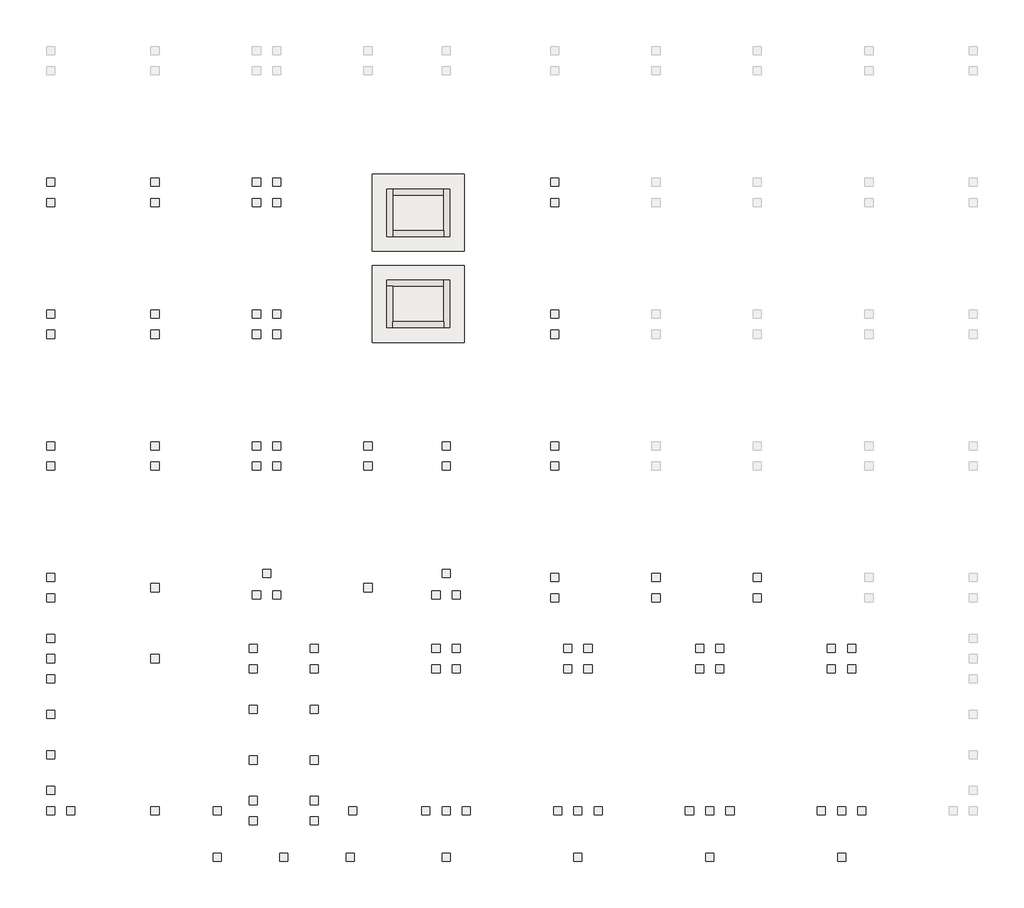
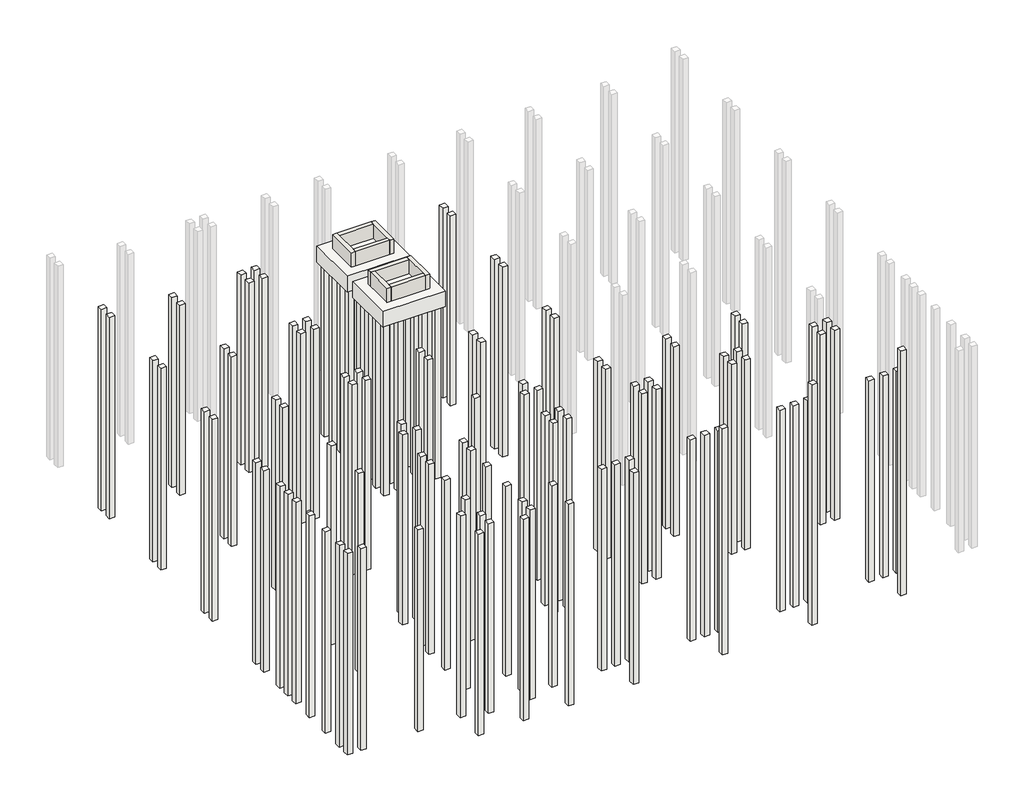
# Not in any storey, part 1 of 2: 143 footings, 8 walls.
# Revit data of these elements (continued)
# Type "NLRS_17_SFO_TLB_funderingspaal geheid beton prefab-AV-MMBPC_gen_rsf : heipaal beton prefab_gen__bxh 400x400"
#   IfcExportAs = "IfcPile"
#   Type Comments = "prefab heipaal 400x400"
#   Model = " "
#   Manufacturer = " "
#   Description = "prefab heipaal 400x400"
#   Assembly Code = "17.21"
#   Width = 400 mm
#   Slanted Angle [instance default] = 0.00°
#   NLRS_S_draagvermogen_trek [instance default] = 0.00 kN
#   NLRS_S_draagvermogen_druk [instance default] = 0.00 kN
#   NLRS_C_lengte [instance default] = 1660 mm
#   NLRS_C_hoogte = 400 mm
#   NLRS_C_breedte = 400 mm
#   Height [instance default] = 1660 mm
#   Length [instance default] = 1660 mm
#   Angle [instance default] = 0.00°
#   Slanted [instance default] = 0
#   Structural Material = NLRS_f2_beton prefab_gen_rsf
#   Keynote = ""
# Type "NLRS_16_WA_beton ihw 300_gen_rsf"
#   Keynote = ""
#   Type IfcGUID = "3S1HfGygHC08_ZXeiJ7DHR"
#   Description = "buitenwand beton ihw, generiek"
#   Assembly Code = "16.23"
#   IfcExportAs = "IfcWall"
#   Layers, outside or top first: 300 mm "NLRS_f2_beton ihwg_gen_rsf" (function 1)
# Element 1 (IfcFooting, "NLRS_16_SFO_LB_funderingspoer meerpaals beton ihwg-MMBC-SH_gen_rsf : funderingspoer beton ihwg_gen__lift bxlxh 3800x4550x1200")
#   IfcGUID = "22y6L5gAz9AR8RjJaZzOwK"
#   Height = 1200 mm
#   Depth = 0 mm
#   IsExternal = yes
#   LoadBearing = yes
#   Phase Created = NLRS_nieuw
#   Materials on its faces: "NLRS_f2_beton ihwg_gen_rsf"
# Element 2 (IfcFooting, "NLRS_16_SFO_LB_funderingspoer meerpaals beton ihwg-MMBC-SH_gen_rsf : funderingspoer beton ihwg_gen__lift bxlxh 3800x4550x1200")
#   IfcGUID = "22y6L5gAz9AR8RjJaZzOui"
#   Height = 1200 mm
#   Depth = 0 mm
#   IsExternal = yes
#   LoadBearing = yes
#   Phase Created = NLRS_nieuw
#   Materials on its faces: "NLRS_f2_beton ihwg_gen_rsf"
# Element 3 (IfcFooting, "NLRS_17_SFO_TLB_funderingspaal geheid beton prefab-AV-MMBPC_gen_rsf : heipaal beton prefab_gen__bxh 400x400")
#   IfcGUID = "10$Kfo5uPCAOPJEOo5LEvz"
#   Slanted Angle = 0.00°
#   NLRS_S_draagvermogen_trek = 0.00 kN
#   NLRS_S_draagvermogen_druk = 0.00 kN
#   Angle = 0.00°
#   IsExternal = yes
#   LoadBearing = yes
#   Slanted = 0
#   Phase Created = NLRS_nieuw
#   Materials on its faces: "NLRS_f2_beton prefab_gen_rsf"
# Element 4 (IfcFooting, "NLRS_17_SFO_TLB_funderingspaal geheid beton prefab-AV-MMBPC_gen_rsf : heipaal beton prefab_gen__bxh 400x400")
#   IfcGUID = "10$Kfo5uPCAOPJEOo5LEuK"
#   Slanted Angle = 0.00°
#   NLRS_S_draagvermogen_trek = 0.00 kN
#   NLRS_S_draagvermogen_druk = 0.00 kN
#   Angle = 0.00°
#   IsExternal = yes
#   LoadBearing = yes
#   Slanted = 0
#   Phase Created = NLRS_nieuw
#   Materials on its faces: "NLRS_f2_beton prefab_gen_rsf"
# Element 5 (IfcFooting, "NLRS_17_SFO_TLB_funderingspaal geheid beton prefab-AV-MMBPC_gen_rsf : heipaal beton prefab_gen__bxh 400x400")
#   IfcGUID = "10$Kfo5uPCAOPJEOo5LEuY"
#   Slanted Angle = 0.00°
#   NLRS_S_draagvermogen_trek = 0.00 kN
#   NLRS_S_draagvermogen_druk = 0.00 kN
#   Angle = 0.00°
#   IsExternal = yes
#   LoadBearing = yes
#   Slanted = 0
#   Phase Created = NLRS_nieuw
#   Materials on its faces: "NLRS_f2_beton prefab_gen_rsf"
# Element 6 (IfcFooting, "NLRS_17_SFO_TLB_funderingspaal geheid beton prefab-AV-MMBPC_gen_rsf : heipaal beton prefab_gen__bxh 400x400")
#   IfcGUID = "10$Kfo5uPCAOPJEOo5LEu$"
#   Slanted Angle = 0.00°
#   NLRS_S_draagvermogen_trek = 0.00 kN
#   NLRS_S_draagvermogen_druk = 0.00 kN
#   Angle = 0.00°
#   IsExternal = yes
#   LoadBearing = yes
#   Slanted = 0
#   Phase Created = NLRS_nieuw
#   Materials on its faces: "NLRS_f2_beton prefab_gen_rsf"
# Element 7 (IfcFooting, "NLRS_17_SFO_TLB_funderingspaal geheid beton prefab-AV-MMBPC_gen_rsf : heipaal beton prefab_gen__bxh 400x400")
#   IfcGUID = "10$Kfo5uPCAOPJEOo5LEun"
#   Slanted Angle = 0.00°
#   NLRS_S_draagvermogen_trek = 0.00 kN
#   NLRS_S_draagvermogen_druk = 0.00 kN
#   Angle = 0.00°
#   IsExternal = yes
#   LoadBearing = yes
#   Slanted = 0
#   Phase Created = NLRS_nieuw
#   Materials on its faces: "NLRS_f2_beton prefab_gen_rsf"
# Element 8 (IfcFooting, "NLRS_17_SFO_TLB_funderingspaal geheid beton prefab-AV-MMBPC_gen_rsf : heipaal beton prefab_gen__bxh 400x400")
#   IfcGUID = "10$Kfo5uPCAOPJEOo5LEtC"
#   Slanted Angle = 0.00°
#   NLRS_S_draagvermogen_trek = 0.00 kN
#   NLRS_S_draagvermogen_druk = 0.00 kN
#   Angle = 0.00°
#   IsExternal = yes
#   LoadBearing = yes
#   Slanted = 0
#   Phase Created = NLRS_nieuw
#   Materials on its faces: "NLRS_f2_beton prefab_gen_rsf"
# Element 9 (IfcFooting, "NLRS_17_SFO_TLB_funderingspaal geheid beton prefab-AV-MMBPC_gen_rsf : heipaal beton prefab_gen__bxh 400x400")
#   IfcGUID = "10$Kfo5uPCAOPJEOo5LEtE"
#   Slanted Angle = 0.00°
#   NLRS_S_draagvermogen_trek = 0.00 kN
#   NLRS_S_draagvermogen_druk = 0.00 kN
#   Angle = 0.00°
#   IsExternal = yes
#   LoadBearing = yes
#   Slanted = 0
#   Phase Created = NLRS_nieuw
#   Materials on its faces: "NLRS_f2_beton prefab_gen_rsf"
# Element 10 (IfcFooting, "NLRS_17_SFO_TLB_funderingspaal geheid beton prefab-AV-MMBPC_gen_rsf : heipaal beton prefab_gen__bxh 400x400")
#   IfcGUID = "10$Kfo5uPCAOPJEOo5LEtR"
#   Slanted Angle = 0.00°
#   NLRS_S_draagvermogen_trek = 0.00 kN
#   NLRS_S_draagvermogen_druk = 0.00 kN
#   Angle = 0.00°
#   IsExternal = yes
#   LoadBearing = yes
#   Slanted = 0
#   Phase Created = NLRS_nieuw
#   Materials on its faces: "NLRS_f2_beton prefab_gen_rsf"
# Element 11 (IfcFooting, "NLRS_17_SFO_TLB_funderingspaal geheid beton prefab-AV-MMBPC_gen_rsf : heipaal beton prefab_gen__bxh 400x400")
#   IfcGUID = "10$Kfo5uPCAOPJEOo5LEtT"
#   Slanted Angle = 0.00°
#   NLRS_S_draagvermogen_trek = 0.00 kN
#   NLRS_S_draagvermogen_druk = 0.00 kN
#   Angle = 0.00°
#   IsExternal = yes
#   LoadBearing = yes
#   Slanted = 0
#   Phase Created = NLRS_nieuw
#   Materials on its faces: "NLRS_f2_beton prefab_gen_rsf"
# Element 12 (IfcFooting, "NLRS_17_SFO_TLB_funderingspaal geheid beton prefab-AV-MMBPC_gen_rsf : heipaal beton prefab_gen__bxh 400x400")
#   IfcGUID = "10$Kfo5uPCAOPJEOo5LEte"
#   Slanted Angle = 0.00°
#   NLRS_S_draagvermogen_trek = 0.00 kN
#   NLRS_S_draagvermogen_druk = 0.00 kN
#   Angle = 0.00°
#   IsExternal = yes
#   LoadBearing = yes
#   Slanted = 0
#   Phase Created = NLRS_nieuw
#   Materials on its faces: "NLRS_f2_beton prefab_gen_rsf"
# Element 13 (IfcFooting, "NLRS_17_SFO_TLB_funderingspaal geheid beton prefab-AV-MMBPC_gen_rsf : heipaal beton prefab_gen__bxh 400x400")
#   IfcGUID = "10$Kfo5uPCAOPJEOo5LEtg"
#   Slanted Angle = 0.00°
#   NLRS_S_draagvermogen_trek = 0.00 kN
#   NLRS_S_draagvermogen_druk = 0.00 kN
#   Angle = 0.00°
#   IsExternal = yes
#   LoadBearing = yes
#   Slanted = 0
#   Phase Created = NLRS_nieuw
#   Materials on its faces: "NLRS_f2_beton prefab_gen_rsf"
# Element 14 (IfcFooting, "NLRS_17_SFO_TLB_funderingspaal geheid beton prefab-AV-MMBPC_gen_rsf : heipaal beton prefab_gen__bxh 400x400")
#   IfcGUID = "10$Kfo5uPCAOPJEOo5LEtb"
#   Slanted Angle = 0.00°
#   NLRS_S_draagvermogen_trek = 0.00 kN
#   NLRS_S_draagvermogen_druk = 0.00 kN
#   Angle = 0.00°
#   IsExternal = yes
#   LoadBearing = yes
#   Slanted = 0
#   Phase Created = NLRS_nieuw
#   Materials on its faces: "NLRS_f2_beton prefab_gen_rsf"
# Element 15 (IfcFooting, "NLRS_17_SFO_TLB_funderingspaal geheid beton prefab-AV-MMBPC_gen_rsf : heipaal beton prefab_gen__bxh 400x400")
#   IfcGUID = "10$Kfo5uPCAOPJEOo5LEtd"
#   Slanted Angle = 0.00°
#   NLRS_S_draagvermogen_trek = 0.00 kN
#   NLRS_S_draagvermogen_druk = 0.00 kN
#   Angle = 0.00°
#   IsExternal = yes
#   LoadBearing = yes
#   Slanted = 0
#   Phase Created = NLRS_nieuw
#   Materials on its faces: "NLRS_f2_beton prefab_gen_rsf"
# Element 16 (IfcFooting, "NLRS_17_SFO_TLB_funderingspaal geheid beton prefab-AV-MMBPC_gen_rsf : heipaal beton prefab_gen__bxh 400x400")
#   IfcGUID = "10$Kfo5uPCAOPJEOo5LEsp"
#   Slanted Angle = 0.00°
#   NLRS_S_draagvermogen_trek = 0.00 kN
#   NLRS_S_draagvermogen_druk = 0.00 kN
#   Angle = 0.00°
#   IsExternal = yes
#   LoadBearing = yes
#   Slanted = 0
#   Phase Created = NLRS_nieuw
#   Materials on its faces: "NLRS_f2_beton prefab_gen_rsf"
# Element 17 (IfcFooting, "NLRS_17_SFO_TLB_funderingspaal geheid beton prefab-AV-MMBPC_gen_rsf : heipaal beton prefab_gen__bxh 400x400")
#   IfcGUID = "10$Kfo5uPCAOPJEOo5LEsr"
#   Slanted Angle = 0.00°
#   NLRS_S_draagvermogen_trek = 0.00 kN
#   NLRS_S_draagvermogen_druk = 0.00 kN
#   Angle = 0.00°
#   IsExternal = yes
#   LoadBearing = yes
#   Slanted = 0
#   Phase Created = NLRS_nieuw
#   Materials on its faces: "NLRS_f2_beton prefab_gen_rsf"
# Element 18 (IfcFooting, "NLRS_17_SFO_TLB_funderingspaal geheid beton prefab-AV-MMBPC_gen_rsf : heipaal beton prefab_gen__bxh 400x400")
#   IfcGUID = "10$Kfo5uPCAOPJEOo5LEr0"
#   Slanted Angle = 0.00°
#   NLRS_S_draagvermogen_trek = 0.00 kN
#   NLRS_S_draagvermogen_druk = 0.00 kN
#   Angle = 0.00°
#   IsExternal = yes
#   LoadBearing = yes
#   Slanted = 0
#   Phase Created = NLRS_nieuw
#   Materials on its faces: "NLRS_f2_beton prefab_gen_rsf"
# Element 19 (IfcFooting, "NLRS_17_SFO_TLB_funderingspaal geheid beton prefab-AV-MMBPC_gen_rsf : heipaal beton prefab_gen__bxh 400x400")
#   IfcGUID = "10$Kfo5uPCAOPJEOo5LEr2"
#   Slanted Angle = 0.00°
#   NLRS_S_draagvermogen_trek = 0.00 kN
#   NLRS_S_draagvermogen_druk = 0.00 kN
#   Angle = 0.00°
#   IsExternal = yes
#   LoadBearing = yes
#   Slanted = 0
#   Phase Created = NLRS_nieuw
#   Materials on its faces: "NLRS_f2_beton prefab_gen_rsf"
# Element 20 (IfcFooting, "NLRS_17_SFO_TLB_funderingspaal geheid beton prefab-AV-MMBPC_gen_rsf : heipaal beton prefab_gen__bxh 400x400")
#   IfcGUID = "10$Kfo5uPCAOPJEOo5LErR"
#   Slanted Angle = 0.00°
#   NLRS_S_draagvermogen_trek = 0.00 kN
#   NLRS_S_draagvermogen_druk = 0.00 kN
#   Angle = 0.00°
#   IsExternal = yes
#   LoadBearing = yes
#   Slanted = 0
#   Phase Created = NLRS_nieuw
#   Materials on its faces: "NLRS_f2_beton prefab_gen_rsf"
# Element 21 (IfcFooting, "NLRS_17_SFO_TLB_funderingspaal geheid beton prefab-AV-MMBPC_gen_rsf : heipaal beton prefab_gen__bxh 400x400")
#   IfcGUID = "10$Kfo5uPCAOPJEOo5LErT"
#   Slanted Angle = 0.00°
#   NLRS_S_draagvermogen_trek = 0.00 kN
#   NLRS_S_draagvermogen_druk = 0.00 kN
#   Angle = 0.00°
#   IsExternal = yes
#   LoadBearing = yes
#   Slanted = 0
#   Phase Created = NLRS_nieuw
#   Materials on its faces: "NLRS_f2_beton prefab_gen_rsf"
# Element 22 (IfcFooting, "NLRS_17_SFO_TLB_funderingspaal geheid beton prefab-AV-MMBPC_gen_rsf : heipaal beton prefab_gen__bxh 400x400")
#   IfcGUID = "10$Kfo5uPCAOPJEOo5LErd"
#   Slanted Angle = 0.00°
#   NLRS_S_draagvermogen_trek = 0.00 kN
#   NLRS_S_draagvermogen_druk = 0.00 kN
#   Angle = 0.00°
#   IsExternal = yes
#   LoadBearing = yes
#   Slanted = 0
#   Phase Created = NLRS_nieuw
#   Materials on its faces: "NLRS_f2_beton prefab_gen_rsf"
# Element 23 (IfcFooting, "NLRS_17_SFO_TLB_funderingspaal geheid beton prefab-AV-MMBPC_gen_rsf : heipaal beton prefab_gen__bxh 400x400")
#   IfcGUID = "10$Kfo5uPCAOPJEOo5LErv"
#   Slanted Angle = 0.00°
#   NLRS_S_draagvermogen_trek = 0.00 kN
#   NLRS_S_draagvermogen_druk = 0.00 kN
#   Angle = 0.00°
#   IsExternal = yes
#   LoadBearing = yes
#   Slanted = 0
#   Phase Created = NLRS_nieuw
#   Materials on its faces: "NLRS_f2_beton prefab_gen_rsf"
# Element 24 (IfcFooting, "NLRS_17_SFO_TLB_funderingspaal geheid beton prefab-AV-MMBPC_gen_rsf : heipaal beton prefab_gen__bxh 400x400")
#   IfcGUID = "10$Kfo5uPCAOPJEOo5LEq5"
#   Slanted Angle = 0.00°
#   NLRS_S_draagvermogen_trek = 0.00 kN
#   NLRS_S_draagvermogen_druk = 0.00 kN
#   Angle = 0.00°
#   IsExternal = yes
#   LoadBearing = yes
#   Slanted = 0
#   Phase Created = NLRS_nieuw
#   Materials on its faces: "NLRS_f2_beton prefab_gen_rsf"
# Element 25 (IfcFooting, "NLRS_17_SFO_TLB_funderingspaal geheid beton prefab-AV-MMBPC_gen_rsf : heipaal beton prefab_gen__bxh 400x400")
#   IfcGUID = "10$Kfo5uPCAOPJEOo5LEq7"
#   Slanted Angle = 0.00°
#   NLRS_S_draagvermogen_trek = 0.00 kN
#   NLRS_S_draagvermogen_druk = 0.00 kN
#   Angle = 0.00°
#   IsExternal = yes
#   LoadBearing = yes
#   Slanted = 0
#   Phase Created = NLRS_nieuw
#   Materials on its faces: "NLRS_f2_beton prefab_gen_rsf"
# Element 26 (IfcFooting, "NLRS_17_SFO_TLB_funderingspaal geheid beton prefab-AV-MMBPC_gen_rsf : heipaal beton prefab_gen__bxh 400x400")
#   IfcGUID = "10$Kfo5uPCAOPJEOo5LEqa"
#   Slanted Angle = 0.00°
#   NLRS_S_draagvermogen_trek = 0.00 kN
#   NLRS_S_draagvermogen_druk = 0.00 kN
#   Angle = 0.00°
#   IsExternal = yes
#   LoadBearing = yes
#   Slanted = 0
#   Phase Created = NLRS_nieuw
#   Materials on its faces: "NLRS_f2_beton prefab_gen_rsf"
# Element 27 (IfcFooting, "NLRS_17_SFO_TLB_funderingspaal geheid beton prefab-AV-MMBPC_gen_rsf : heipaal beton prefab_gen__bxh 400x400")
#   IfcGUID = "10$Kfo5uPCAOPJEOo5LEqc"
#   Slanted Angle = 0.00°
#   NLRS_S_draagvermogen_trek = 0.00 kN
#   NLRS_S_draagvermogen_druk = 0.00 kN
#   Angle = 0.00°
#   IsExternal = yes
#   LoadBearing = yes
#   Slanted = 0
#   Phase Created = NLRS_nieuw
#   Materials on its faces: "NLRS_f2_beton prefab_gen_rsf"
# Element 28 (IfcFooting, "NLRS_17_SFO_TLB_funderingspaal geheid beton prefab-AV-MMBPC_gen_rsf : heipaal beton prefab_gen__bxh 400x400")
#   IfcGUID = "10$Kfo5uPCAOPJEOo5LEqy"
#   Slanted Angle = 0.00°
#   NLRS_S_draagvermogen_trek = 0.00 kN
#   NLRS_S_draagvermogen_druk = 0.00 kN
#   Angle = 0.00°
#   IsExternal = yes
#   LoadBearing = yes
#   Slanted = 0
#   Phase Created = NLRS_nieuw
#   Materials on its faces: "NLRS_f2_beton prefab_gen_rsf"
# Element 29 (IfcFooting, "NLRS_17_SFO_TLB_funderingspaal geheid beton prefab-AV-MMBPC_gen_rsf : heipaal beton prefab_gen__bxh 400x400")
#   IfcGUID = "10$Kfo5uPCAOPJEOo5LEq_"
#   Slanted Angle = 0.00°
#   NLRS_S_draagvermogen_trek = 0.00 kN
#   NLRS_S_draagvermogen_druk = 0.00 kN
#   Angle = 0.00°
#   IsExternal = yes
#   LoadBearing = yes
#   Slanted = 0
#   Phase Created = NLRS_nieuw
#   Materials on its faces: "NLRS_f2_beton prefab_gen_rsf"
# Element 30 (IfcFooting, "NLRS_17_SFO_TLB_funderingspaal geheid beton prefab-AV-MMBPC_gen_rsf : heipaal beton prefab_gen__bxh 400x400")
#   IfcGUID = "10$Kfo5uPCAOPJEOo5LEpB"
#   Slanted Angle = 0.00°
#   NLRS_S_draagvermogen_trek = 0.00 kN
#   NLRS_S_draagvermogen_druk = 0.00 kN
#   Angle = 0.00°
#   IsExternal = yes
#   LoadBearing = yes
#   Slanted = 0
#   Phase Created = NLRS_nieuw
#   Materials on its faces: "NLRS_f2_beton prefab_gen_rsf"
# Element 31 (IfcFooting, "NLRS_17_SFO_TLB_funderingspaal geheid beton prefab-AV-MMBPC_gen_rsf : heipaal beton prefab_gen__bxh 400x400")
#   IfcGUID = "10$Kfo5uPCAOPJEOo5LEpD"
#   Slanted Angle = 0.00°
#   NLRS_S_draagvermogen_trek = 0.00 kN
#   NLRS_S_draagvermogen_druk = 0.00 kN
#   Angle = 0.00°
#   IsExternal = yes
#   LoadBearing = yes
#   Slanted = 0
#   Phase Created = NLRS_nieuw
#   Materials on its faces: "NLRS_f2_beton prefab_gen_rsf"
# Element 32 (IfcFooting, "NLRS_17_SFO_TLB_funderingspaal geheid beton prefab-AV-MMBPC_gen_rsf : heipaal beton prefab_gen__bxh 400x400")
#   IfcGUID = "10$Kfo5uPCAOPJEOo5LEp3"
#   Slanted Angle = 0.00°
#   NLRS_S_draagvermogen_trek = 0.00 kN
#   NLRS_S_draagvermogen_druk = 0.00 kN
#   Angle = 0.00°
#   IsExternal = yes
#   LoadBearing = yes
#   Slanted = 0
#   Phase Created = NLRS_nieuw
#   Materials on its faces: "NLRS_f2_beton prefab_gen_rsf"
# Element 33 (IfcFooting, "NLRS_17_SFO_TLB_funderingspaal geheid beton prefab-AV-MMBPC_gen_rsf : heipaal beton prefab_gen__bxh 400x400")
#   IfcGUID = "10$Kfo5uPCAOPJEOo5LEp5"
#   Slanted Angle = 0.00°
#   NLRS_S_draagvermogen_trek = 0.00 kN
#   NLRS_S_draagvermogen_druk = 0.00 kN
#   Angle = 0.00°
#   IsExternal = yes
#   LoadBearing = yes
#   Slanted = 0
#   Phase Created = NLRS_nieuw
#   Materials on its faces: "NLRS_f2_beton prefab_gen_rsf"
# Element 34 (IfcFooting, "NLRS_17_SFO_TLB_funderingspaal geheid beton prefab-AV-MMBPC_gen_rsf : heipaal beton prefab_gen__bxh 400x400")
#   IfcGUID = "10$Kfo5uPCAOPJEOo5LEpG"
#   Slanted Angle = 0.00°
#   NLRS_S_draagvermogen_trek = 0.00 kN
#   NLRS_S_draagvermogen_druk = 0.00 kN
#   Angle = 0.00°
#   IsExternal = yes
#   LoadBearing = yes
#   Slanted = 0
#   Phase Created = NLRS_nieuw
#   Materials on its faces: "NLRS_f2_beton prefab_gen_rsf"
# Element 35 (IfcFooting, "NLRS_17_SFO_TLB_funderingspaal geheid beton prefab-AV-MMBPC_gen_rsf : heipaal beton prefab_gen__bxh 400x400")
#   IfcGUID = "10$Kfo5uPCAOPJEOo5LEpI"
#   Slanted Angle = 0.00°
#   NLRS_S_draagvermogen_trek = 0.00 kN
#   NLRS_S_draagvermogen_druk = 0.00 kN
#   Angle = 0.00°
#   IsExternal = yes
#   LoadBearing = yes
#   Slanted = 0
#   Phase Created = NLRS_nieuw
#   Materials on its faces: "NLRS_f2_beton prefab_gen_rsf"
# Element 36 (IfcFooting, "NLRS_17_SFO_TLB_funderingspaal geheid beton prefab-AV-MMBPC_gen_rsf : heipaal beton prefab_gen__bxh 400x400")
#   IfcGUID = "10$Kfo5uPCAOPJEOo5LEpe"
#   Slanted Angle = 0.00°
#   NLRS_S_draagvermogen_trek = 0.00 kN
#   NLRS_S_draagvermogen_druk = 0.00 kN
#   Angle = 0.00°
#   IsExternal = yes
#   LoadBearing = yes
#   Slanted = 0
#   Phase Created = NLRS_nieuw
#   Materials on its faces: "NLRS_f2_beton prefab_gen_rsf"
# Element 37 (IfcFooting, "NLRS_17_SFO_TLB_funderingspaal geheid beton prefab-AV-MMBPC_gen_rsf : heipaal beton prefab_gen__bxh 400x400")
#   IfcGUID = "10$Kfo5uPCAOPJEOo5LEpg"
#   Slanted Angle = 0.00°
#   NLRS_S_draagvermogen_trek = 0.00 kN
#   NLRS_S_draagvermogen_druk = 0.00 kN
#   Angle = 0.00°
#   IsExternal = yes
#   LoadBearing = yes
#   Slanted = 0
#   Phase Created = NLRS_nieuw
#   Materials on its faces: "NLRS_f2_beton prefab_gen_rsf"
# Element 38 (IfcFooting, "NLRS_17_SFO_TLB_funderingspaal geheid beton prefab-AV-MMBPC_gen_rsf : heipaal beton prefab_gen__bxh 400x400")
#   IfcGUID = "10$Kfo5uPCAOPJEOo5LEoA"
#   Slanted Angle = 0.00°
#   NLRS_S_draagvermogen_trek = 0.00 kN
#   NLRS_S_draagvermogen_druk = 0.00 kN
#   Angle = 0.00°
#   IsExternal = yes
#   LoadBearing = yes
#   Slanted = 0
#   Phase Created = NLRS_nieuw
#   Materials on its faces: "NLRS_f2_beton prefab_gen_rsf"
# Element 39 (IfcFooting, "NLRS_17_SFO_TLB_funderingspaal geheid beton prefab-AV-MMBPC_gen_rsf : heipaal beton prefab_gen__bxh 400x400")
#   IfcGUID = "10$Kfo5uPCAOPJEOo5LEoC"
#   Slanted Angle = 0.00°
#   NLRS_S_draagvermogen_trek = 0.00 kN
#   NLRS_S_draagvermogen_druk = 0.00 kN
#   Angle = 0.00°
#   IsExternal = yes
#   LoadBearing = yes
#   Slanted = 0
#   Phase Created = NLRS_nieuw
#   Materials on its faces: "NLRS_f2_beton prefab_gen_rsf"
# Element 40 (IfcFooting, "NLRS_17_SFO_TLB_funderingspaal geheid beton prefab-AV-MMBPC_gen_rsf : heipaal beton prefab_gen__bxh 400x400")
#   IfcGUID = "10$Kfo5uPCAOPJEOo5LEo2"
#   Slanted Angle = 0.00°
#   NLRS_S_draagvermogen_trek = 0.00 kN
#   NLRS_S_draagvermogen_druk = 0.00 kN
#   Angle = 0.00°
#   IsExternal = yes
#   LoadBearing = yes
#   Slanted = 0
#   Phase Created = NLRS_nieuw
#   Materials on its faces: "NLRS_f2_beton prefab_gen_rsf"
# Element 41 (IfcFooting, "NLRS_17_SFO_TLB_funderingspaal geheid beton prefab-AV-MMBPC_gen_rsf : heipaal beton prefab_gen__bxh 400x400")
#   IfcGUID = "10$Kfo5uPCAOPJEOo5LEo4"
#   Slanted Angle = 0.00°
#   NLRS_S_draagvermogen_trek = 0.00 kN
#   NLRS_S_draagvermogen_druk = 0.00 kN
#   Angle = 0.00°
#   IsExternal = yes
#   LoadBearing = yes
#   Slanted = 0
#   Phase Created = NLRS_nieuw
#   Materials on its faces: "NLRS_f2_beton prefab_gen_rsf"
# Element 42 (IfcFooting, "NLRS_17_SFO_TLB_funderingspaal geheid beton prefab-AV-MMBPC_gen_rsf : heipaal beton prefab_gen__bxh 400x400")
#   IfcGUID = "10$Kfo5uPCAOPJEOo5LEoV"
#   Slanted Angle = 0.00°
#   NLRS_S_draagvermogen_trek = 0.00 kN
#   NLRS_S_draagvermogen_druk = 0.00 kN
#   Angle = 0.00°
#   IsExternal = yes
#   LoadBearing = yes
#   Slanted = 0
#   Phase Created = NLRS_nieuw
#   Materials on its faces: "NLRS_f2_beton prefab_gen_rsf"
# Element 43 (IfcFooting, "NLRS_17_SFO_TLB_funderingspaal geheid beton prefab-AV-MMBPC_gen_rsf : heipaal beton prefab_gen__bxh 400x400")
#   IfcGUID = "10$Kfo5uPCAOPJEOo5LEoH"
#   Slanted Angle = 0.00°
#   NLRS_S_draagvermogen_trek = 0.00 kN
#   NLRS_S_draagvermogen_druk = 0.00 kN
#   Angle = 0.00°
#   IsExternal = yes
#   LoadBearing = yes
#   Slanted = 0
#   Phase Created = NLRS_nieuw
#   Materials on its faces: "NLRS_f2_beton prefab_gen_rsf"
# Element 44 (IfcFooting, "NLRS_17_SFO_TLB_funderingspaal geheid beton prefab-AV-MMBPC_gen_rsf : heipaal beton prefab_gen__bxh 400x400")
#   IfcGUID = "10$Kfo5uPCAOPJEOo5LEoN"
#   Slanted Angle = 0.00°
#   NLRS_S_draagvermogen_trek = 0.00 kN
#   NLRS_S_draagvermogen_druk = 0.00 kN
#   Angle = 0.00°
#   IsExternal = yes
#   LoadBearing = yes
#   Slanted = 0
#   Phase Created = NLRS_nieuw
#   Materials on its faces: "NLRS_f2_beton prefab_gen_rsf"
# Element 45 (IfcFooting, "NLRS_17_SFO_TLB_funderingspaal geheid beton prefab-AV-MMBPC_gen_rsf : heipaal beton prefab_gen__bxh 400x400")
#   IfcGUID = "10$Kfo5uPCAOPJEOo5LEof"
#   Slanted Angle = 0.00°
#   NLRS_S_draagvermogen_trek = 0.00 kN
#   NLRS_S_draagvermogen_druk = 0.00 kN
#   Angle = 0.00°
#   IsExternal = yes
#   LoadBearing = yes
#   Slanted = 0
#   Phase Created = NLRS_nieuw
#   Materials on its faces: "NLRS_f2_beton prefab_gen_rsf"
# Element 46 (IfcFooting, "NLRS_17_SFO_TLB_funderingspaal geheid beton prefab-AV-MMBPC_gen_rsf : heipaal beton prefab_gen__bxh 400x400")
#   IfcGUID = "10$Kfo5uPCAOPJEOo5LEoc"
#   Slanted Angle = 0.00°
#   NLRS_S_draagvermogen_trek = 0.00 kN
#   NLRS_S_draagvermogen_druk = 0.00 kN
#   Angle = 0.00°
#   IsExternal = yes
#   LoadBearing = yes
#   Slanted = 0
#   Phase Created = NLRS_nieuw
#   Materials on its faces: "NLRS_f2_beton prefab_gen_rsf"
# Element 47 (IfcFooting, "NLRS_17_SFO_TLB_funderingspaal geheid beton prefab-AV-MMBPC_gen_rsf : heipaal beton prefab_gen__bxh 400x400")
#   IfcGUID = "10$Kfo5uPCAOPJEOo5LEou"
#   Slanted Angle = 0.00°
#   NLRS_S_draagvermogen_trek = 0.00 kN
#   NLRS_S_draagvermogen_druk = 0.00 kN
#   Angle = 0.00°
#   IsExternal = yes
#   LoadBearing = yes
#   Slanted = 0
#   Phase Created = NLRS_nieuw
#   Materials on its faces: "NLRS_f2_beton prefab_gen_rsf"
# Element 48 (IfcFooting, "NLRS_17_SFO_TLB_funderingspaal geheid beton prefab-AV-MMBPC_gen_rsf : heipaal beton prefab_gen__bxh 400x400")
#   IfcGUID = "10$Kfo5uPCAOPJEOo5LEo_"
#   Slanted Angle = 0.00°
#   NLRS_S_draagvermogen_trek = 0.00 kN
#   NLRS_S_draagvermogen_druk = 0.00 kN
#   Angle = 0.00°
#   IsExternal = yes
#   LoadBearing = yes
#   Slanted = 0
#   Phase Created = NLRS_nieuw
#   Materials on its faces: "NLRS_f2_beton prefab_gen_rsf"
# Element 49 (IfcFooting, "NLRS_17_SFO_TLB_funderingspaal geheid beton prefab-AV-MMBPC_gen_rsf : heipaal beton prefab_gen__bxh 400x400")
#   IfcGUID = "10$Kfo5uPCAOPJEOo5LEom"
#   Slanted Angle = 0.00°
#   NLRS_S_draagvermogen_trek = 0.00 kN
#   NLRS_S_draagvermogen_druk = 0.00 kN
#   Angle = 0.00°
#   IsExternal = yes
#   LoadBearing = yes
#   Slanted = 0
#   Phase Created = NLRS_nieuw
#   Materials on its faces: "NLRS_f2_beton prefab_gen_rsf"
# Element 50 (IfcFooting, "NLRS_17_SFO_TLB_funderingspaal geheid beton prefab-AV-MMBPC_gen_rsf : heipaal beton prefab_gen__bxh 400x400")
#   IfcGUID = "10$Kfo5uPCAOPJEOo5LEnB"
#   Slanted Angle = 0.00°
#   NLRS_S_draagvermogen_trek = 0.00 kN
#   NLRS_S_draagvermogen_druk = 0.00 kN
#   Angle = 0.00°
#   IsExternal = yes
#   LoadBearing = yes
#   Slanted = 0
#   Phase Created = NLRS_nieuw
#   Materials on its faces: "NLRS_f2_beton prefab_gen_rsf"
# Element 51 (IfcFooting, "NLRS_17_SFO_TLB_funderingspaal geheid beton prefab-AV-MMBPC_gen_rsf : heipaal beton prefab_gen__bxh 400x400")
#   IfcGUID = "10$Kfo5uPCAOPJEOo5LEnF"
#   Slanted Angle = 0.00°
#   NLRS_S_draagvermogen_trek = 0.00 kN
#   NLRS_S_draagvermogen_druk = 0.00 kN
#   Angle = 0.00°
#   IsExternal = yes
#   LoadBearing = yes
#   Slanted = 0
#   Phase Created = NLRS_nieuw
#   Materials on its faces: "NLRS_f2_beton prefab_gen_rsf"
# Element 52 (IfcFooting, "NLRS_17_SFO_TLB_funderingspaal geheid beton prefab-AV-MMBPC_gen_rsf : heipaal beton prefab_gen__bxh 400x400")
#   IfcGUID = "10$Kfo5uPCAOPJEOo5LEn1"
#   Slanted Angle = 0.00°
#   NLRS_S_draagvermogen_trek = 0.00 kN
#   NLRS_S_draagvermogen_druk = 0.00 kN
#   Angle = 0.00°
#   IsExternal = yes
#   LoadBearing = yes
#   Slanted = 0
#   Phase Created = NLRS_nieuw
#   Materials on its faces: "NLRS_f2_beton prefab_gen_rsf"
# Element 53 (IfcFooting, "NLRS_17_SFO_TLB_funderingspaal geheid beton prefab-AV-MMBPC_gen_rsf : heipaal beton prefab_gen__bxh 400x400")
#   IfcGUID = "10$Kfo5uPCAOPJEOo5LEWk"
#   Slanted Angle = 0.00°
#   NLRS_S_draagvermogen_trek = 0.00 kN
#   NLRS_S_draagvermogen_druk = 0.00 kN
#   Angle = 0.00°
#   IsExternal = yes
#   LoadBearing = yes
#   Slanted = 0
#   Phase Created = NLRS_nieuw
#   Materials on its faces: "NLRS_f2_beton prefab_gen_rsf"
# Element 54 (IfcFooting, "NLRS_17_SFO_TLB_funderingspaal geheid beton prefab-AV-MMBPC_gen_rsf : heipaal beton prefab_gen__bxh 400x400")
#   IfcGUID = "10$Kfo5uPCAOPJEOo5LEWW"
#   Slanted Angle = 0.00°
#   NLRS_S_draagvermogen_trek = 0.00 kN
#   NLRS_S_draagvermogen_druk = 0.00 kN
#   Angle = 0.00°
#   IsExternal = yes
#   LoadBearing = yes
#   Slanted = 0
#   Phase Created = NLRS_nieuw
#   Materials on its faces: "NLRS_f2_beton prefab_gen_rsf"
# Element 55 (IfcFooting, "NLRS_17_SFO_TLB_funderingspaal geheid beton prefab-AV-MMBPC_gen_rsf : heipaal beton prefab_gen__bxh 400x400")
#   IfcGUID = "10$Kfo5uPCAOPJEOo5LEWY"
#   Slanted Angle = 0.00°
#   NLRS_S_draagvermogen_trek = 0.00 kN
#   NLRS_S_draagvermogen_druk = 0.00 kN
#   Angle = 0.00°
#   IsExternal = yes
#   LoadBearing = yes
#   Slanted = 0
#   Phase Created = NLRS_nieuw
#   Materials on its faces: "NLRS_f2_beton prefab_gen_rsf"
# Element 56 (IfcFooting, "NLRS_17_SFO_TLB_funderingspaal geheid beton prefab-AV-MMBPC_gen_rsf : heipaal beton prefab_gen__bxh 400x400")
#   IfcGUID = "10$Kfo5uPCAOPJEOo5LEWa"
#   Slanted Angle = 0.00°
#   NLRS_S_draagvermogen_trek = 0.00 kN
#   NLRS_S_draagvermogen_druk = 0.00 kN
#   Angle = 0.00°
#   IsExternal = yes
#   LoadBearing = yes
#   Slanted = 0
#   Phase Created = NLRS_nieuw
#   Materials on its faces: "NLRS_f2_beton prefab_gen_rsf"
# Element 57 (IfcFooting, "NLRS_17_SFO_TLB_funderingspaal geheid beton prefab-AV-MMBPC_gen_rsf : heipaal beton prefab_gen__bxh 400x400")
#   IfcGUID = "10$Kfo5uPCAOPJEOo5LEWp"
#   Slanted Angle = 0.00°
#   NLRS_S_draagvermogen_trek = 0.00 kN
#   NLRS_S_draagvermogen_druk = 0.00 kN
#   Angle = 0.00°
#   IsExternal = yes
#   LoadBearing = yes
#   Slanted = 0
#   Phase Created = NLRS_nieuw
#   Materials on its faces: "NLRS_f2_beton prefab_gen_rsf"
# Element 58 (IfcFooting, "NLRS_17_SFO_TLB_funderingspaal geheid beton prefab-AV-MMBPC_gen_rsf : heipaal beton prefab_gen__bxh 400x400")
#   IfcGUID = "10$Kfo5uPCAOPJEOo5LEWr"
#   Slanted Angle = 0.00°
#   NLRS_S_draagvermogen_trek = 0.00 kN
#   NLRS_S_draagvermogen_druk = 0.00 kN
#   Angle = 0.00°
#   IsExternal = yes
#   LoadBearing = yes
#   Slanted = 0
#   Phase Created = NLRS_nieuw
#   Materials on its faces: "NLRS_f2_beton prefab_gen_rsf"
# Element 59 (IfcFooting, "NLRS_17_SFO_TLB_funderingspaal geheid beton prefab-AV-MMBPC_gen_rsf : heipaal beton prefab_gen__bxh 400x400")
#   IfcGUID = "10$Kfo5uPCAOPJEOo5LEWt"
#   Slanted Angle = 0.00°
#   NLRS_S_draagvermogen_trek = 0.00 kN
#   NLRS_S_draagvermogen_druk = 0.00 kN
#   Angle = 0.00°
#   IsExternal = yes
#   LoadBearing = yes
#   Slanted = 0
#   Phase Created = NLRS_nieuw
#   Materials on its faces: "NLRS_f2_beton prefab_gen_rsf"
# Element 60 (IfcFooting, "NLRS_17_SFO_TLB_funderingspaal geheid beton prefab-AV-MMBPC_gen_rsf : heipaal beton prefab_gen__bxh 400x400")
#   IfcGUID = "10$Kfo5uPCAOPJEOo5LFV9"
#   Slanted Angle = 0.00°
#   NLRS_S_draagvermogen_trek = 0.00 kN
#   NLRS_S_draagvermogen_druk = 0.00 kN
#   Angle = 0.00°
#   IsExternal = yes
#   LoadBearing = yes
#   Slanted = 0
#   Phase Created = NLRS_nieuw
#   Materials on its faces: "NLRS_f2_beton prefab_gen_rsf"
# Element 61 (IfcFooting, "NLRS_17_SFO_TLB_funderingspaal geheid beton prefab-AV-MMBPC_gen_rsf : heipaal beton prefab_gen__bxh 400x400")
#   IfcGUID = "10$Kfo5uPCAOPJEOo5LFVh"
#   Slanted Angle = 0.00°
#   NLRS_S_draagvermogen_trek = 0.00 kN
#   NLRS_S_draagvermogen_druk = 0.00 kN
#   Angle = 0.00°
#   IsExternal = yes
#   LoadBearing = yes
#   Slanted = 0
#   Phase Created = NLRS_nieuw
#   Materials on its faces: "NLRS_f2_beton prefab_gen_rsf"
# Element 62 (IfcFooting, "NLRS_17_SFO_TLB_funderingspaal geheid beton prefab-AV-MMBPC_gen_rsf : heipaal beton prefab_gen__bxh 400x400")
#   IfcGUID = "10$Kfo5uPCAOPJEOo5LFNw"
#   Slanted Angle = 0.00°
#   NLRS_S_draagvermogen_trek = 0.00 kN
#   NLRS_S_draagvermogen_druk = 0.00 kN
#   Angle = 0.00°
#   IsExternal = yes
#   LoadBearing = yes
#   Slanted = 0
#   Phase Created = NLRS_nieuw
#   Materials on its faces: "NLRS_f2_beton prefab_gen_rsf"
# Element 63 (IfcFooting, "NLRS_17_SFO_TLB_funderingspaal geheid beton prefab-AV-MMBPC_gen_rsf : heipaal beton prefab_gen__bxh 400x400")
#   IfcGUID = "0NibaB7BP2RgdAc9dAk1VF"
#   Slanted Angle = 0.00°
#   NLRS_S_draagvermogen_trek = 0.00 kN
#   NLRS_S_draagvermogen_druk = 0.00 kN
#   Angle = 0.00°
#   IsExternal = yes
#   LoadBearing = yes
#   Slanted = 0
#   Phase Created = NLRS_nieuw
#   Materials on its faces: "NLRS_f2_beton prefab_gen_rsf"
# Element 64 (IfcFooting, "NLRS_17_SFO_TLB_funderingspaal geheid beton prefab-AV-MMBPC_gen_rsf : heipaal beton prefab_gen__bxh 400x400")
#   IfcGUID = "0NibaB7BP2RgdAc9dAk1UY"
#   Slanted Angle = 0.00°
#   NLRS_S_draagvermogen_trek = 0.00 kN
#   NLRS_S_draagvermogen_druk = 0.00 kN
#   Angle = 0.00°
#   IsExternal = yes
#   LoadBearing = yes
#   Slanted = 0
#   Phase Created = NLRS_nieuw
#   Materials on its faces: "NLRS_f2_beton prefab_gen_rsf"
# Element 65 (IfcFooting, "NLRS_17_SFO_TLB_funderingspaal geheid beton prefab-AV-MMBPC_gen_rsf : heipaal beton prefab_gen__bxh 400x400")
#   IfcGUID = "3loy75XKz2Rw4dS8JWiauf"
#   Slanted Angle = 0.00°
#   NLRS_S_draagvermogen_trek = 0.00 kN
#   NLRS_S_draagvermogen_druk = 0.00 kN
#   Angle = 0.00°
#   IsExternal = yes
#   LoadBearing = yes
#   Slanted = 0
#   Phase Created = NLRS_nieuw
#   Materials on its faces: "NLRS_f2_beton prefab_gen_rsf"
# Element 66 (IfcFooting, "NLRS_17_SFO_TLB_funderingspaal geheid beton prefab-AV-MMBPC_gen_rsf : heipaal beton prefab_gen__bxh 400x400")
#   IfcGUID = "3loy75XKz2Rw4dS8JWiaul"
#   Slanted Angle = 0.00°
#   NLRS_S_draagvermogen_trek = 0.00 kN
#   NLRS_S_draagvermogen_druk = 0.00 kN
#   Angle = 0.00°
#   IsExternal = yes
#   LoadBearing = yes
#   Slanted = 0
#   Phase Created = NLRS_nieuw
#   Materials on its faces: "NLRS_f2_beton prefab_gen_rsf"
# Element 67 (IfcFooting, "NLRS_17_SFO_TLB_funderingspaal geheid beton prefab-AV-MMBPC_gen_rsf : heipaal beton prefab_gen__bxh 400x400")
#   IfcGUID = "3loy75XKz2Rw4dS8JWiauj"
#   Slanted Angle = 0.00°
#   NLRS_S_draagvermogen_trek = 0.00 kN
#   NLRS_S_draagvermogen_druk = 0.00 kN
#   Angle = 0.00°
#   IsExternal = yes
#   LoadBearing = yes
#   Slanted = 0
#   Phase Created = NLRS_nieuw
#   Materials on its faces: "NLRS_f2_beton prefab_gen_rsf"
# Element 68 (IfcFooting, "NLRS_17_SFO_TLB_funderingspaal geheid beton prefab-AV-MMBPC_gen_rsf : heipaal beton prefab_gen__bxh 400x400")
#   IfcGUID = "3loy75XKz2Rw4dS8JWiam3"
#   Slanted Angle = 0.00°
#   NLRS_S_draagvermogen_trek = 0.00 kN
#   NLRS_S_draagvermogen_druk = 0.00 kN
#   Angle = 0.00°
#   IsExternal = yes
#   LoadBearing = yes
#   Slanted = 0
#   Phase Created = NLRS_nieuw
#   Materials on its faces: "NLRS_f2_beton prefab_gen_rsf"
# Element 69 (IfcFooting, "NLRS_17_SFO_TLB_funderingspaal geheid beton prefab-AV-MMBPC_gen_rsf : heipaal beton prefab_gen__bxh 400x400")
#   IfcGUID = "3loy75XKz2Rw4dS8JWiam1"
#   Slanted Angle = 0.00°
#   NLRS_S_draagvermogen_trek = 0.00 kN
#   NLRS_S_draagvermogen_druk = 0.00 kN
#   Angle = 0.00°
#   IsExternal = yes
#   LoadBearing = yes
#   Slanted = 0
#   Phase Created = NLRS_nieuw
#   Materials on its faces: "NLRS_f2_beton prefab_gen_rsf"
# Element 70 (IfcFooting, "NLRS_17_SFO_TLB_funderingspaal geheid beton prefab-AV-MMBPC_gen_rsf : heipaal beton prefab_gen__bxh 400x400")
#   IfcGUID = "3loy75XKz2Rw4dS8JWiapu"
#   Slanted Angle = 0.00°
#   NLRS_S_draagvermogen_trek = 0.00 kN
#   NLRS_S_draagvermogen_druk = 0.00 kN
#   Angle = 0.00°
#   IsExternal = yes
#   LoadBearing = yes
#   Slanted = 0
#   Phase Created = NLRS_nieuw
#   Materials on its faces: "NLRS_f2_beton prefab_gen_rsf"
# Element 71 (IfcFooting, "NLRS_17_SFO_TLB_funderingspaal geheid beton prefab-AV-MMBPC_gen_rsf : heipaal beton prefab_gen__bxh 400x400")
#   IfcGUID = "3loy75XKz2Rw4dS8JWiap_"
#   Slanted Angle = 0.00°
#   NLRS_S_draagvermogen_trek = 0.00 kN
#   NLRS_S_draagvermogen_druk = 0.00 kN
#   Angle = 0.00°
#   IsExternal = yes
#   LoadBearing = yes
#   Slanted = 0
#   Phase Created = NLRS_nieuw
#   Materials on its faces: "NLRS_f2_beton prefab_gen_rsf"
# Element 72 (IfcFooting, "NLRS_17_SFO_TLB_funderingspaal geheid beton prefab-AV-MMBPC_gen_rsf : heipaal beton prefab_gen__bxh 400x400")
#   IfcGUID = "3loy75XKz2Rw4dS8JWiaoR"
#   Slanted Angle = 0.00°
#   NLRS_S_draagvermogen_trek = 0.00 kN
#   NLRS_S_draagvermogen_druk = 0.00 kN
#   Angle = 0.00°
#   IsExternal = yes
#   LoadBearing = yes
#   Slanted = 0
#   Phase Created = NLRS_nieuw
#   Materials on its faces: "NLRS_f2_beton prefab_gen_rsf"
# Element 73 (IfcFooting, "NLRS_17_SFO_TLB_funderingspaal geheid beton prefab-AV-MMBPC_gen_rsf : heipaal beton prefab_gen__bxh 400x400")
#   IfcGUID = "3loy75XKz2Rw4dS8JWiaoP"
#   Slanted Angle = 0.00°
#   NLRS_S_draagvermogen_trek = 0.00 kN
#   NLRS_S_draagvermogen_druk = 0.00 kN
#   Angle = 0.00°
#   IsExternal = yes
#   LoadBearing = yes
#   Slanted = 0
#   Phase Created = NLRS_nieuw
#   Materials on its faces: "NLRS_f2_beton prefab_gen_rsf"
# Element 74 (IfcFooting, "NLRS_17_SFO_TLB_funderingspaal geheid beton prefab-AV-MMBPC_gen_rsf : heipaal beton prefab_gen__bxh 400x400")
#   IfcGUID = "0NibaB7BP2RgdAc9dAk1EY"
#   Slanted Angle = 0.00°
#   NLRS_S_draagvermogen_trek = 0.00 kN
#   NLRS_S_draagvermogen_druk = 0.00 kN
#   Angle = 0.00°
#   IsExternal = yes
#   LoadBearing = yes
#   Slanted = 0
#   Phase Created = NLRS_nieuw
#   Materials on its faces: "NLRS_f2_beton prefab_gen_rsf"
# Element 75 (IfcFooting, "NLRS_17_SFO_TLB_funderingspaal geheid beton prefab-AV-MMBPC_gen_rsf : heipaal beton prefab_gen__bxh 400x400")
#   IfcGUID = "0NibaB7BP2RgdAc9dAk1EP"
#   Slanted Angle = 0.00°
#   NLRS_S_draagvermogen_trek = 0.00 kN
#   NLRS_S_draagvermogen_druk = 0.00 kN
#   Angle = 0.00°
#   IsExternal = yes
#   LoadBearing = yes
#   Slanted = 0
#   Phase Created = NLRS_nieuw
#   Materials on its faces: "NLRS_f2_beton prefab_gen_rsf"
# Element 76 (IfcFooting, "NLRS_17_SFO_TLB_funderingspaal geheid beton prefab-AV-MMBPC_gen_rsf : heipaal beton prefab_gen__bxh 400x400")
#   IfcGUID = "0NibaB7BP2RgdAc9dAk1Di"
#   Slanted Angle = 0.00°
#   NLRS_S_draagvermogen_trek = 0.00 kN
#   NLRS_S_draagvermogen_druk = 0.00 kN
#   Angle = 0.00°
#   IsExternal = yes
#   LoadBearing = yes
#   Slanted = 0
#   Phase Created = NLRS_nieuw
#   Materials on its faces: "NLRS_f2_beton prefab_gen_rsf"
# Element 77 (IfcFooting, "NLRS_17_SFO_TLB_funderingspaal geheid beton prefab-AV-MMBPC_gen_rsf : heipaal beton prefab_gen__bxh 400x400")
#   IfcGUID = "0NibaB7BP2RgdAc9dAk1SD"
#   Slanted Angle = 0.00°
#   NLRS_S_draagvermogen_trek = 0.00 kN
#   NLRS_S_draagvermogen_druk = 0.00 kN
#   Angle = 0.00°
#   IsExternal = yes
#   LoadBearing = yes
#   Slanted = 0
#   Phase Created = NLRS_nieuw
#   Materials on its faces: "NLRS_f2_beton prefab_gen_rsf"
# Element 78 (IfcFooting, "NLRS_17_SFO_TLB_funderingspaal geheid beton prefab-AV-MMBPC_gen_rsf : heipaal beton prefab_gen__bxh 400x400")
#   IfcGUID = "0NibaB7BP2RgdAc9dAk6Zm"
#   Slanted Angle = 0.00°
#   NLRS_S_draagvermogen_trek = 0.00 kN
#   NLRS_S_draagvermogen_druk = 0.00 kN
#   Angle = 0.00°
#   IsExternal = yes
#   LoadBearing = yes
#   Slanted = 0
#   Phase Created = NLRS_nieuw
#   Materials on its faces: "NLRS_f2_beton prefab_gen_rsf"
# Element 79 (IfcFooting, "NLRS_17_SFO_TLB_funderingspaal geheid beton prefab-AV-MMBPC_gen_rsf : heipaal beton prefab_gen__bxh 400x400")
#   IfcGUID = "0NibaB7BP2RgdAc9dAk6ZH"
#   Slanted Angle = 0.00°
#   NLRS_S_draagvermogen_trek = 0.00 kN
#   NLRS_S_draagvermogen_druk = 0.00 kN
#   Angle = 0.00°
#   IsExternal = yes
#   LoadBearing = yes
#   Slanted = 0
#   Phase Created = NLRS_nieuw
#   Materials on its faces: "NLRS_f2_beton prefab_gen_rsf"
# Element 80 (IfcFooting, "NLRS_17_SFO_TLB_funderingspaal geheid beton prefab-AV-MMBPC_gen_rsf : heipaal beton prefab_gen__bxh 400x400")
#   IfcGUID = "0NibaB7BP2RgdAc9dAk6Y9"
#   Slanted Angle = 0.00°
#   NLRS_S_draagvermogen_trek = 0.00 kN
#   NLRS_S_draagvermogen_druk = 0.00 kN
#   Angle = 0.00°
#   IsExternal = yes
#   LoadBearing = yes
#   Slanted = 0
#   Phase Created = NLRS_nieuw
#   Materials on its faces: "NLRS_f2_beton prefab_gen_rsf"
# Element 81 (IfcFooting, "NLRS_17_SFO_TLB_funderingspaal geheid beton prefab-AV-MMBPC_gen_rsf : heipaal beton prefab_gen__bxh 400x400")
#   IfcGUID = "0NibaB7BP2RgdAc9dAk6Y7"
#   Slanted Angle = 0.00°
#   NLRS_S_draagvermogen_trek = 0.00 kN
#   NLRS_S_draagvermogen_druk = 0.00 kN
#   Angle = 0.00°
#   IsExternal = yes
#   LoadBearing = yes
#   Slanted = 0
#   Phase Created = NLRS_nieuw
#   Materials on its faces: "NLRS_f2_beton prefab_gen_rsf"
# Element 82 (IfcFooting, "NLRS_17_SFO_TLB_funderingspaal geheid beton prefab-AV-MMBPC_gen_rsf : heipaal beton prefab_gen__bxh 400x400")
#   IfcGUID = "0NibaB7BP2RgdAc9dAk6XN"
#   Slanted Angle = 0.00°
#   NLRS_S_draagvermogen_trek = 0.00 kN
#   NLRS_S_draagvermogen_druk = 0.00 kN
#   Angle = 0.00°
#   IsExternal = yes
#   LoadBearing = yes
#   Slanted = 0
#   Phase Created = NLRS_nieuw
#   Materials on its faces: "NLRS_f2_beton prefab_gen_rsf"
# Element 83 (IfcFooting, "NLRS_17_SFO_TLB_funderingspaal geheid beton prefab-AV-MMBPC_gen_rsf : heipaal beton prefab_gen__bxh 400x400")
#   IfcGUID = "0NibaB7BP2RgdAc9dAk6Wo"
#   Slanted Angle = 0.00°
#   NLRS_S_draagvermogen_trek = 0.00 kN
#   NLRS_S_draagvermogen_druk = 0.00 kN
#   Angle = 0.00°
#   IsExternal = yes
#   LoadBearing = yes
#   Slanted = 0
#   Phase Created = NLRS_nieuw
#   Materials on its faces: "NLRS_f2_beton prefab_gen_rsf"
# Element 84 (IfcFooting, "NLRS_17_SFO_TLB_funderingspaal geheid beton prefab-AV-MMBPC_gen_rsf : heipaal beton prefab_gen__bxh 400x400")
#   IfcGUID = "0NibaB7BP2RgdAc9dAk6a5"
#   Slanted Angle = 0.00°
#   NLRS_S_draagvermogen_trek = 0.00 kN
#   NLRS_S_draagvermogen_druk = 0.00 kN
#   Angle = 0.00°
#   IsExternal = yes
#   LoadBearing = yes
#   Slanted = 0
#   Phase Created = NLRS_nieuw
#   Materials on its faces: "NLRS_f2_beton prefab_gen_rsf"
# Element 85 (IfcFooting, "NLRS_17_SFO_TLB_funderingspaal geheid beton prefab-AV-MMBPC_gen_rsf : heipaal beton prefab_gen__bxh 400x400")
#   IfcGUID = "0NibaB7BP2RgdAc9dAk6aO"
#   Slanted Angle = 0.00°
#   NLRS_S_draagvermogen_trek = 0.00 kN
#   NLRS_S_draagvermogen_druk = 0.00 kN
#   Angle = 0.00°
#   IsExternal = yes
#   LoadBearing = yes
#   Slanted = 0
#   Phase Created = NLRS_nieuw
#   Materials on its faces: "NLRS_f2_beton prefab_gen_rsf"
# Element 86 (IfcFooting, "NLRS_17_SFO_TLB_funderingspaal geheid beton prefab-AV-MMBPC_gen_rsf : heipaal beton prefab_gen__bxh 400x400")
#   IfcGUID = "0NibaB7BP2RgdAc9dAk6hl"
#   Slanted Angle = 0.00°
#   NLRS_S_draagvermogen_trek = 0.00 kN
#   NLRS_S_draagvermogen_druk = 0.00 kN
#   Angle = 0.00°
#   IsExternal = yes
#   LoadBearing = yes
#   Slanted = 0
#   Phase Created = NLRS_nieuw
#   Materials on its faces: "NLRS_f2_beton prefab_gen_rsf"
# Element 87 (IfcFooting, "NLRS_17_SFO_TLB_funderingspaal geheid beton prefab-AV-MMBPC_gen_rsf : heipaal beton prefab_gen__bxh 400x400")
#   IfcGUID = "0NibaB7BP2RgdAc9dAk6hr"
#   Slanted Angle = 0.00°
#   NLRS_S_draagvermogen_trek = 0.00 kN
#   NLRS_S_draagvermogen_druk = 0.00 kN
#   Angle = 0.00°
#   IsExternal = yes
#   LoadBearing = yes
#   Slanted = 0
#   Phase Created = NLRS_nieuw
#   Materials on its faces: "NLRS_f2_beton prefab_gen_rsf"
# Element 88 (IfcFooting, "NLRS_17_SFO_TLB_funderingspaal geheid beton prefab-AV-MMBPC_gen_rsf : heipaal beton prefab_gen__bxh 400x400")
#   IfcGUID = "0NibaB7BP2RgdAc9dAk6hp"
#   Slanted Angle = 0.00°
#   NLRS_S_draagvermogen_trek = 0.00 kN
#   NLRS_S_draagvermogen_druk = 0.00 kN
#   Angle = 0.00°
#   IsExternal = yes
#   LoadBearing = yes
#   Slanted = 0
#   Phase Created = NLRS_nieuw
#   Materials on its faces: "NLRS_f2_beton prefab_gen_rsf"
# Element 89 (IfcFooting, "NLRS_17_SFO_TLB_funderingspaal geheid beton prefab-AV-MMBPC_gen_rsf : heipaal beton prefab_gen__bxh 400x400")
#   IfcGUID = "0NibaB7BP2RgdAc9dAk6hn"
#   Slanted Angle = 0.00°
#   NLRS_S_draagvermogen_trek = 0.00 kN
#   NLRS_S_draagvermogen_druk = 0.00 kN
#   Angle = 0.00°
#   IsExternal = yes
#   LoadBearing = yes
#   Slanted = 0
#   Phase Created = NLRS_nieuw
#   Materials on its faces: "NLRS_f2_beton prefab_gen_rsf"
# Element 90 (IfcFooting, "NLRS_17_SFO_TLB_funderingspaal geheid beton prefab-AV-MMBPC_gen_rsf : heipaal beton prefab_gen__bxh 400x400")
#   IfcGUID = "0NibaB7BP2RgdAc9dAk6h2"
#   Slanted Angle = 0.00°
#   NLRS_S_draagvermogen_trek = 0.00 kN
#   NLRS_S_draagvermogen_druk = 0.00 kN
#   Angle = 0.00°
#   IsExternal = yes
#   LoadBearing = yes
#   Slanted = 0
#   Phase Created = NLRS_nieuw
#   Materials on its faces: "NLRS_f2_beton prefab_gen_rsf"
# Element 91 (IfcFooting, "NLRS_17_SFO_TLB_funderingspaal geheid beton prefab-AV-MMBPC_gen_rsf : heipaal beton prefab_gen__bxh 400x400")
#   IfcGUID = "0NibaB7BP2RgdAc9dAk6h0"
#   Slanted Angle = 0.00°
#   NLRS_S_draagvermogen_trek = 0.00 kN
#   NLRS_S_draagvermogen_druk = 0.00 kN
#   Angle = 0.00°
#   IsExternal = yes
#   LoadBearing = yes
#   Slanted = 0
#   Phase Created = NLRS_nieuw
#   Materials on its faces: "NLRS_f2_beton prefab_gen_rsf"
# Element 92 (IfcFooting, "NLRS_17_SFO_TLB_funderingspaal geheid beton prefab-AV-MMBPC_gen_rsf : heipaal beton prefab_gen__bxh 400x400")
#   IfcGUID = "0NibaB7BP2RgdAc9dAk6hU"
#   Slanted Angle = 0.00°
#   NLRS_S_draagvermogen_trek = 0.00 kN
#   NLRS_S_draagvermogen_druk = 0.00 kN
#   Angle = 0.00°
#   IsExternal = yes
#   LoadBearing = yes
#   Slanted = 0
#   Phase Created = NLRS_nieuw
#   Materials on its faces: "NLRS_f2_beton prefab_gen_rsf"
# Element 93 (IfcFooting, "NLRS_17_SFO_TLB_funderingspaal geheid beton prefab-AV-MMBPC_gen_rsf : heipaal beton prefab_gen__bxh 400x400")
#   IfcGUID = "0NibaB7BP2RgdAc9dAk6hN"
#   Slanted Angle = 0.00°
#   NLRS_S_draagvermogen_trek = 0.00 kN
#   NLRS_S_draagvermogen_druk = 0.00 kN
#   Angle = 0.00°
#   IsExternal = yes
#   LoadBearing = yes
#   Slanted = 0
#   Phase Created = NLRS_nieuw
#   Materials on its faces: "NLRS_f2_beton prefab_gen_rsf"
# Element 94 (IfcFooting, "NLRS_17_SFO_TLB_funderingspaal geheid beton prefab-AV-MMBPC_gen_rsf : heipaal beton prefab_gen__bxh 400x400")
#   IfcGUID = "0NibaB7BP2RgdAc9dAk6hL"
#   Slanted Angle = 0.00°
#   NLRS_S_draagvermogen_trek = 0.00 kN
#   NLRS_S_draagvermogen_druk = 0.00 kN
#   Angle = 0.00°
#   IsExternal = yes
#   LoadBearing = yes
#   Slanted = 0
#   Phase Created = NLRS_nieuw
#   Materials on its faces: "NLRS_f2_beton prefab_gen_rsf"
# Element 95 (IfcFooting, "NLRS_17_SFO_TLB_funderingspaal geheid beton prefab-AV-MMBPC_gen_rsf : heipaal beton prefab_gen__bxh 400x400")
#   IfcGUID = "0NibaB7BP2RgdAc9dAk6hJ"
#   Slanted Angle = 0.00°
#   NLRS_S_draagvermogen_trek = 0.00 kN
#   NLRS_S_draagvermogen_druk = 0.00 kN
#   Angle = 0.00°
#   IsExternal = yes
#   LoadBearing = yes
#   Slanted = 0
#   Phase Created = NLRS_nieuw
#   Materials on its faces: "NLRS_f2_beton prefab_gen_rsf"
# Element 96 (IfcFooting, "NLRS_17_SFO_TLB_funderingspaal geheid beton prefab-AV-MMBPC_gen_rsf : heipaal beton prefab_gen__bxh 400x400")
#   IfcGUID = "0NibaB7BP2RgdAc9dAk6gq"
#   Slanted Angle = 0.00°
#   NLRS_S_draagvermogen_trek = 0.00 kN
#   NLRS_S_draagvermogen_druk = 0.00 kN
#   Angle = 0.00°
#   IsExternal = yes
#   LoadBearing = yes
#   Slanted = 0
#   Phase Created = NLRS_nieuw
#   Materials on its faces: "NLRS_f2_beton prefab_gen_rsf"
# Element 97 (IfcFooting, "NLRS_17_SFO_TLB_funderingspaal geheid beton prefab-AV-MMBPC_gen_rsf : heipaal beton prefab_gen__bxh 400x400")
#   IfcGUID = "3loy75XKz2Rw4dS8JWiaWl"
#   Slanted Angle = 0.00°
#   NLRS_S_draagvermogen_trek = 0.00 kN
#   NLRS_S_draagvermogen_druk = 0.00 kN
#   Angle = 0.00°
#   IsExternal = yes
#   LoadBearing = yes
#   Slanted = 0
#   Phase Created = NLRS_nieuw
#   Materials on its faces: "NLRS_f2_beton prefab_gen_rsf"
# Element 98 (IfcFooting, "NLRS_17_SFO_TLB_funderingspaal geheid beton prefab-AV-MMBPC_gen_rsf : heipaal beton prefab_gen__bxh 400x400")
#   IfcGUID = "3loy75XKz2Rw4dS8JWiaZK"
#   Slanted Angle = 0.00°
#   NLRS_S_draagvermogen_trek = 0.00 kN
#   NLRS_S_draagvermogen_druk = 0.00 kN
#   Angle = 0.00°
#   IsExternal = yes
#   LoadBearing = yes
#   Slanted = 0
#   Phase Created = NLRS_nieuw
#   Materials on its faces: "NLRS_f2_beton prefab_gen_rsf"
# Element 99 (IfcFooting, "NLRS_17_SFO_TLB_funderingspaal geheid beton prefab-AV-MMBPC_gen_rsf : heipaal beton prefab_gen__bxh 400x400")
#   IfcGUID = "3loy75XKz2Rw4dS8JWiaqJ"
#   Slanted Angle = 0.00°
#   NLRS_S_draagvermogen_trek = 0.00 kN
#   NLRS_S_draagvermogen_druk = 0.00 kN
#   Angle = 0.00°
#   IsExternal = yes
#   LoadBearing = yes
#   Slanted = 0
#   Phase Created = NLRS_nieuw
#   Materials on its faces: "NLRS_f2_beton prefab_gen_rsf"
